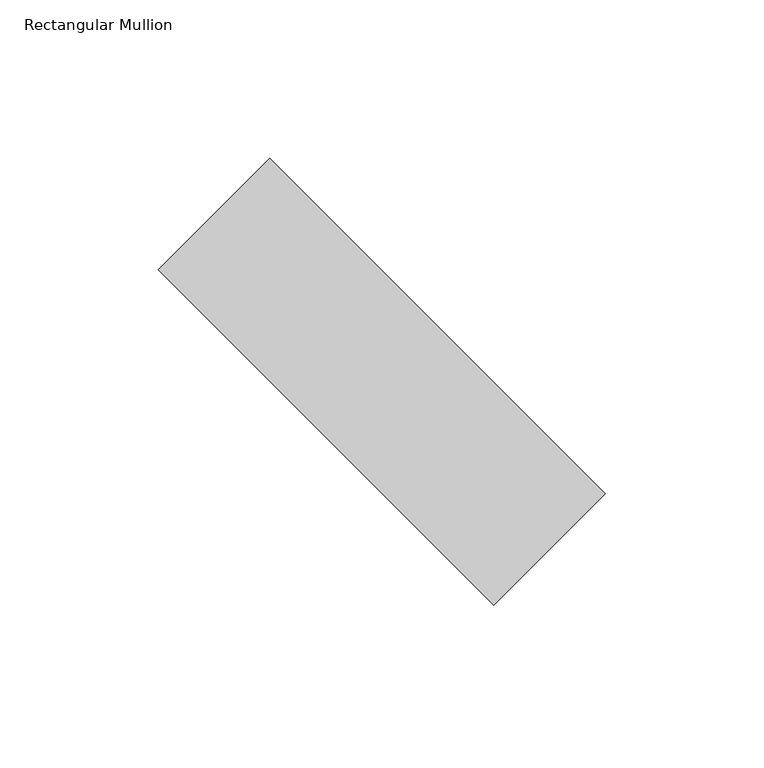
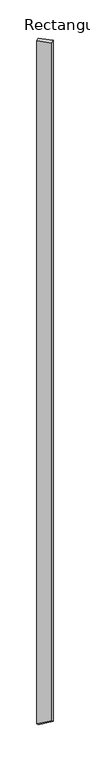
"""IFC4 building model written with IfcOpenShell, lengths in millimetres: member geometry, Rectangular Mullion : tilted mullions."""

from ifc_helpers import new_model, si_unit, origin, place, context, project, spatial, faceted_brep, source, transform, mapped, element, save


def rectangular_mullion_e764de33(model_context):
    return source(origin(), model_context, "Body", "Brep", [
        faceted_brep([(-35.3553391, 70.7106781, 0.0), (-70.7106781, 35.3553391, 0.0), (35.3553391, -70.7106781, 0.0), (70.7106781, -35.3553391, 0.0), (-35.3553391, 70.7106781, -8054.5115791), (-70.7106781, 35.3553391, -8009.4581263), (35.3553391, -70.7106781, -7944.4067811), (70.7106781, -35.3553391, -7989.4602339)], [[[0, 1, 2, 3]], [[1, 0, 4, 5]], [[2, 1, 5, 6]], [[3, 2, 6, 7]], [[0, 3, 7, 4]], [[4, 7, 6, 5]]]),
    ])


if __name__ == "__main__":
    model = new_model("IFC4")
    model_context = context("Model", 3, world=origin())
    ifc_project = project(units=[si_unit("LENGTHUNIT", "METRE", prefix="MILLI")], contexts=[model_context])
    site = spatial("IfcSite", under=ifc_project)
    building = spatial("IfcBuilding", under=site)
    placement = place(None, origin())
    rectangular_mullion_shape = rectangular_mullion_e764de33(model_context)
    element("IfcMember", 1, ObjectType="Rectangular Mullion : tilted mullions", at=placement, inside=building, context=model_context, shape_type="MappedRepresentation", body=[
        mapped(rectangular_mullion_shape, transform((0.0, 0.0, 0.0), x_axis=(1.0, 0.0, 0.0), y_axis=(0.0, 1.0, 0.0), z_axis=(0.0, 0.0, 1.0))),
    ])
    save(model, "model.ifc")

# Revit data of these elements
# Type "Rectangular Mullion : tilted mullions"
#   built-in parameter 1007304 = 0.492126 (stored number, unit not read)
#   built-in parameter 1007301 = 0.082021 (stored number, unit not read)
#   built-in parameter 1007300 = 0.082021 (stored number, unit not read)
# Element 1 (IfcMember, "Rectangular Mullion : tilted mullions")
#   Materials on its faces: "Aluminum"
# Materials
#   "Aluminum": class "Metal", colour RGB 244 244 244, transparency 0, Description = "Aluminum 6061", Cost = 0
